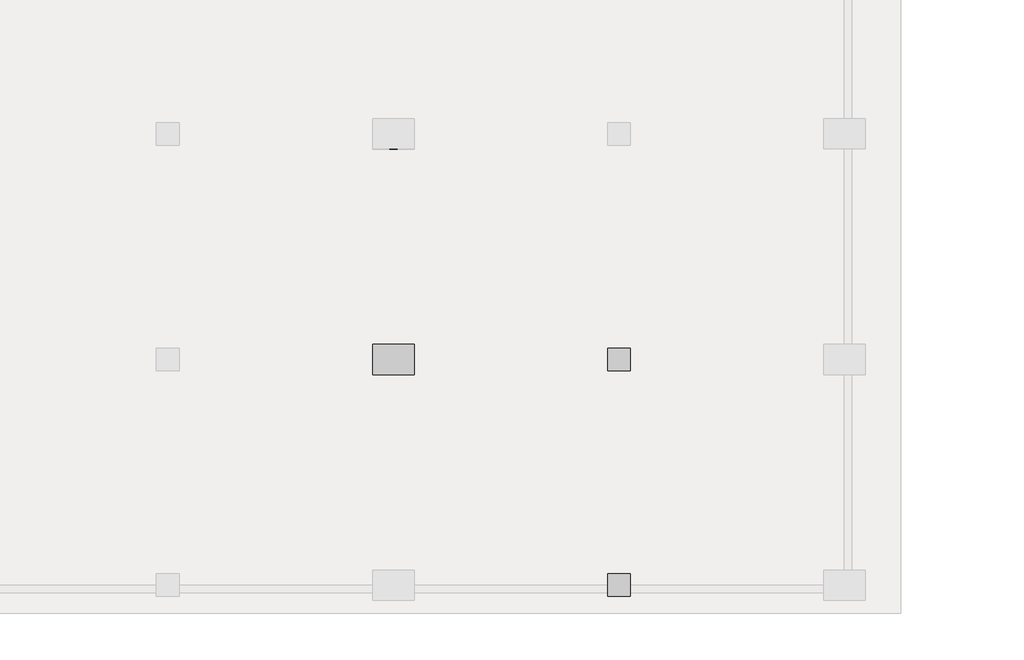
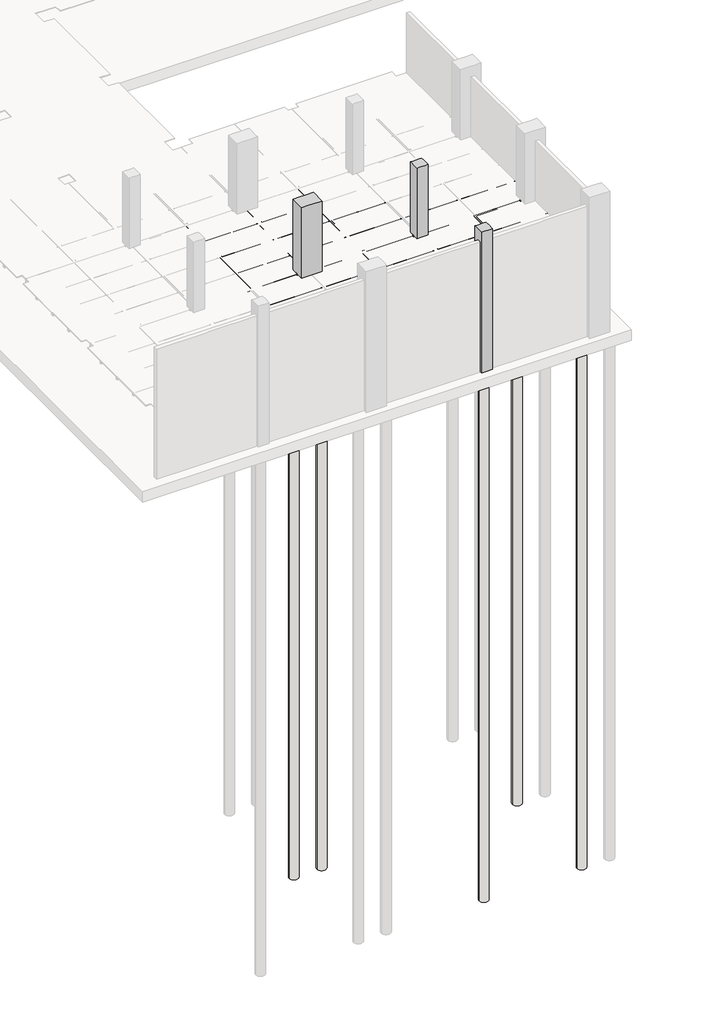
# Not in any storey, part 4 of 16: 30 beams, 5 slabs, 3 columns.
"""IFC4 building model written with IfcOpenShell, lengths in millimetres."""

from ifc_helpers import new_model, si_unit, point, frame, frame_2d, origin, place, context, project, spatial, polyline, circle_curve, trimmed, segment, composite_curve, outline, extrude, faceted_brep, element, save

model = new_model("IFC4")

# Units and contexts
model_context = context("Model", 3, world=origin())
ifc_project = project(units=[si_unit("LENGTHUNIT", "METRE", prefix="MILLI")], contexts=[model_context])

# Site, building
site = spatial("IfcSite", under=ifc_project)
building = spatial("IfcBuilding", under=site)

# Beams
placement = place(None, origin())
element("IfcBeam", 1, ObjectType="Steel Framing_H_KS : H_SB_AR_S02_H-400x200x8x13_BSG1", at=placement, inside=building, context=model_context, shape_type="SweptSolid", body=[
    extrude(outline(composite_curve([segment(polyline([(-53900.0, -4187.0381366), (-53900.0, -4200.0381366), (-54100.0, -4200.0381366), (-54100.0, -4187.0381366), (-54020.0, -4187.0381366)]), True, "CONTINUOUS"), segment(trimmed(circle_curve(frame_2d((-54020.0, -4171.0381366)), 16.0), [point((-54020.0, -4187.0381366))], [point((-54004.0, -4171.0381366))], True, "CARTESIAN"), True, "CONTINUOUS"), segment(polyline([(-54004.0, -4171.0381366), (-54004.0, -3829.0381366)]), True, "CONTINUOUS"), segment(trimmed(circle_curve(frame_2d((-54020.0, -3829.0381366)), 16.0), [point((-54004.0, -3829.0381366))], [point((-54020.0, -3813.0381366))], True, "CARTESIAN"), True, "CONTINUOUS"), segment(polyline([(-54020.0, -3813.0381366), (-54100.0, -3813.0381366), (-54100.0, -3800.0381366), (-53900.0, -3800.0381366), (-53900.0, -3813.0381366), (-53980.0, -3813.0381366)]), True, "CONTINUOUS"), segment(trimmed(circle_curve(frame_2d((-53980.0, -3829.0381366)), 16.0), [point((-53980.0, -3813.0381366))], [point((-53996.0, -3829.0381366))], True, "CARTESIAN"), True, "CONTINUOUS"), segment(polyline([(-53996.0, -3829.0381366), (-53996.0, -4171.0381366)]), True, "CONTINUOUS"), segment(trimmed(circle_curve(frame_2d((-53980.0, -4171.0381366)), 16.0), [point((-53996.0, -4171.0381366))], [point((-53980.0, -4187.0381366))], True, "CARTESIAN"), True, "CONTINUOUS"), segment(polyline([(-53980.0, -4187.0381366), (-53900.0, -4187.0381366)]), True, "CONTINUOUS")], self_intersect=False)), frame((30312.7, 0.0, 0.0), z_axis=(1.0, 0.0, 0.0), x_axis=(0.0, 1.0, 0.0)), (0.0, 0.0, 1.0), 5124.6),
])
element("IfcBeam", 2, ObjectType="Steel Framing_H_KS : H_SB_AR_S02_H-400x200x8x13_BSG2", at=placement, inside=building, context=model_context, shape_type="SweptSolid", body=[
    extrude(outline(composite_curve([segment(polyline([(-4187.0381366, 35900.0), (-4200.0381366, 35900.0), (-4200.0381366, 36100.0), (-4187.0381366, 36100.0), (-4187.0381366, 36020.0)]), True, "CONTINUOUS"), segment(trimmed(circle_curve(frame_2d((-4171.0381366, 36020.0)), 16.0), [point((-4187.0381366, 36020.0))], [point((-4171.0381366, 36004.0))], True, "CARTESIAN"), True, "CONTINUOUS"), segment(polyline([(-4171.0381366, 36004.0), (-3829.0381366, 36004.0)]), True, "CONTINUOUS"), segment(trimmed(circle_curve(frame_2d((-3829.0381366, 36020.0)), 16.0), [point((-3829.0381366, 36004.0))], [point((-3813.0381366, 36020.0))], True, "CARTESIAN"), True, "CONTINUOUS"), segment(polyline([(-3813.0381366, 36020.0), (-3813.0381366, 36100.0), (-3800.0381366, 36100.0), (-3800.0381366, 35900.0), (-3813.0381366, 35900.0), (-3813.0381366, 35980.0)]), True, "CONTINUOUS"), segment(trimmed(circle_curve(frame_2d((-3829.0381366, 35980.0)), 16.0), [point((-3813.0381366, 35980.0))], [point((-3829.0381366, 35996.0))], True, "CARTESIAN"), True, "CONTINUOUS"), segment(polyline([(-3829.0381366, 35996.0), (-4171.0381366, 35996.0)]), True, "CONTINUOUS"), segment(trimmed(circle_curve(frame_2d((-4171.0381366, 35980.0)), 16.0), [point((-4171.0381366, 35996.0))], [point((-4187.0381366, 35980.0))], True, "CARTESIAN"), True, "CONTINUOUS"), segment(polyline([(-4187.0381366, 35980.0), (-4187.0381366, 35900.0)]), True, "CONTINUOUS")], self_intersect=False)), frame((0.0, -53587.3, 0.0), z_axis=(0.0, 1.0, 0.0), x_axis=(0.0, 0.0, 1.0)), (0.0, 0.0, 1.0), 5174.6),
])
element("IfcBeam", 3, ObjectType="Steel Framing_H_KS : H_SB_AR_S02_H-400x200x8x13_BSB1", at=placement, inside=building, context=model_context, shape_type="SweptSolid", body=[
    extrude(outline(composite_curve([segment(polyline([(-4187.0381366, 32900.0), (-4200.0381366, 32900.0), (-4200.0381366, 33100.0), (-4187.0381366, 33100.0), (-4187.0381366, 33020.0)]), True, "CONTINUOUS"), segment(trimmed(circle_curve(frame_2d((-4171.0381366, 33020.0)), 16.0), [point((-4187.0381366, 33020.0))], [point((-4171.0381366, 33004.0))], True, "CARTESIAN"), True, "CONTINUOUS"), segment(polyline([(-4171.0381366, 33004.0), (-3829.0381366, 33004.0)]), True, "CONTINUOUS"), segment(trimmed(circle_curve(frame_2d((-3829.0381366, 33020.0)), 16.0), [point((-3829.0381366, 33004.0))], [point((-3813.0381366, 33020.0))], True, "CARTESIAN"), True, "CONTINUOUS"), segment(polyline([(-3813.0381366, 33020.0), (-3813.0381366, 33100.0), (-3800.0381366, 33100.0), (-3800.0381366, 32900.0), (-3813.0381366, 32900.0), (-3813.0381366, 32980.0)]), True, "CONTINUOUS"), segment(trimmed(circle_curve(frame_2d((-3829.0381366, 32980.0)), 16.0), [point((-3813.0381366, 32980.0))], [point((-3829.0381366, 32996.0))], True, "CARTESIAN"), True, "CONTINUOUS"), segment(polyline([(-3829.0381366, 32996.0), (-4171.0381366, 32996.0)]), True, "CONTINUOUS"), segment(trimmed(circle_curve(frame_2d((-4171.0381366, 32980.0)), 16.0), [point((-4171.0381366, 32996.0))], [point((-4187.0381366, 32980.0))], True, "CARTESIAN"), True, "CONTINUOUS"), segment(polyline([(-4187.0381366, 32980.0), (-4187.0381366, 32900.0)]), True, "CONTINUOUS")], self_intersect=False)), frame((0.0, -53887.3, 0.0), z_axis=(0.0, 1.0, 0.0), x_axis=(0.0, 0.0, 1.0)), (0.0, 0.0, 1.0), 5774.6),
])
element("IfcBeam", 4, ObjectType="Steel Framing_C_KS : H_SB_AR_S02_C-150x75x6.5x10_J1", at=placement, inside=building, context=model_context, shape_type="SweptSolid", body=[
    extrude(outline(composite_curve([segment(polyline([(-50977.2, -3800.0381366), (-50977.2, -3950.0381366), (-51052.2, -3950.0381366)]), True, "CONTINUOUS"), segment(trimmed(circle_curve(frame_2d((-51042.2, -3950.0381366)), 10.0), [point((-51052.2, -3950.0381366))], [point((-51042.2, -3940.0381366))], False, "CARTESIAN"), True, "CONTINUOUS"), segment(polyline([(-51042.2, -3940.0381366), (-50983.7, -3930.7726469), (-50983.7, -3819.3036264), (-51042.2, -3810.0381366)]), True, "CONTINUOUS"), segment(trimmed(circle_curve(frame_2d((-51042.2, -3800.0381366)), 10.0), [point((-51042.2, -3810.0381366))], [point((-51052.2, -3800.0381366))], False, "CARTESIAN"), True, "CONTINUOUS"), segment(polyline([(-51052.2, -3800.0381366), (-50977.2, -3800.0381366)]), True, "CONTINUOUS")], self_intersect=False)), frame((33112.7, 0.0, 0.0), z_axis=(1.0, 0.0, 0.0), x_axis=(0.0, 1.0, 0.0)), (0.0, 0.0, 1.0), 2774.6),
])
element("IfcBeam", 5, ObjectType="Steel Framing_C_KS : H_SB_AR_S02_C-150x75x6.5x10_J1", at=placement, inside=building, context=model_context, shape_type="SweptSolid", body=[
    extrude(outline(composite_curve([segment(polyline([(-52477.2, -3800.0381366), (-52477.2, -3950.0381366), (-52552.2, -3950.0381366)]), True, "CONTINUOUS"), segment(trimmed(circle_curve(frame_2d((-52542.2, -3950.0381366)), 10.0), [point((-52552.2, -3950.0381366))], [point((-52542.2, -3940.0381366))], False, "CARTESIAN"), True, "CONTINUOUS"), segment(polyline([(-52542.2, -3940.0381366), (-52483.7, -3930.7726469), (-52483.7, -3819.3036264), (-52542.2, -3810.0381366)]), True, "CONTINUOUS"), segment(trimmed(circle_curve(frame_2d((-52542.2, -3800.0381366)), 10.0), [point((-52542.2, -3810.0381366))], [point((-52552.2, -3800.0381366))], False, "CARTESIAN"), True, "CONTINUOUS"), segment(polyline([(-52552.2, -3800.0381366), (-52477.2, -3800.0381366)]), True, "CONTINUOUS")], self_intersect=False)), frame((33112.7, 0.0, 0.0), z_axis=(1.0, 0.0, 0.0), x_axis=(0.0, 1.0, 0.0)), (0.0, 0.0, 1.0), 2774.6),
])
element("IfcBeam", 6, ObjectType="Steel Framing_C_KS : H_SB_AR_S02_C-150x75x6.5x10_J1", at=placement, inside=building, context=model_context, shape_type="SweptSolid", body=[
    extrude(outline(composite_curve([segment(polyline([(-49477.2, -3800.0381366), (-49477.2, -3950.0381366), (-49552.2, -3950.0381366)]), True, "CONTINUOUS"), segment(trimmed(circle_curve(frame_2d((-49542.2, -3950.0381366)), 10.0), [point((-49552.2, -3950.0381366))], [point((-49542.2, -3940.0381366))], False, "CARTESIAN"), True, "CONTINUOUS"), segment(polyline([(-49542.2, -3940.0381366), (-49483.7, -3930.7726469), (-49483.7, -3819.3036264), (-49542.2, -3810.0381366)]), True, "CONTINUOUS"), segment(trimmed(circle_curve(frame_2d((-49542.2, -3800.0381366)), 10.0), [point((-49542.2, -3810.0381366))], [point((-49552.2, -3800.0381366))], False, "CARTESIAN"), True, "CONTINUOUS"), segment(polyline([(-49552.2, -3800.0381366), (-49477.2, -3800.0381366)]), True, "CONTINUOUS")], self_intersect=False)), frame((33112.7, 0.0, 0.0), z_axis=(1.0, 0.0, 0.0), x_axis=(0.0, 1.0, 0.0)), (0.0, 0.0, 1.0), 2774.6),
])
element("IfcBeam", 7, ObjectType="Steel Framing_H_KS : H_SB_AR_S02_H-400x200x8x13_BSG1", at=placement, inside=building, context=model_context, shape_type="SweptSolid", body=[
    extrude(outline(composite_curve([segment(polyline([(-53900.0, -4187.0381366), (-53900.0, -4200.0381366), (-54100.0, -4200.0381366), (-54100.0, -4187.0381366), (-54020.0, -4187.0381366)]), True, "CONTINUOUS"), segment(trimmed(circle_curve(frame_2d((-54020.0, -4171.0381366)), 16.0), [point((-54020.0, -4187.0381366))], [point((-54004.0, -4171.0381366))], True, "CARTESIAN"), True, "CONTINUOUS"), segment(polyline([(-54004.0, -4171.0381366), (-54004.0, -3829.0381366)]), True, "CONTINUOUS"), segment(trimmed(circle_curve(frame_2d((-54020.0, -3829.0381366)), 16.0), [point((-54004.0, -3829.0381366))], [point((-54020.0, -3813.0381366))], True, "CARTESIAN"), True, "CONTINUOUS"), segment(polyline([(-54020.0, -3813.0381366), (-54100.0, -3813.0381366), (-54100.0, -3800.0381366), (-53900.0, -3800.0381366), (-53900.0, -3813.0381366), (-53980.0, -3813.0381366)]), True, "CONTINUOUS"), segment(trimmed(circle_curve(frame_2d((-53980.0, -3829.0381366)), 16.0), [point((-53980.0, -3813.0381366))], [point((-53996.0, -3829.0381366))], True, "CARTESIAN"), True, "CONTINUOUS"), segment(polyline([(-53996.0, -3829.0381366), (-53996.0, -4171.0381366)]), True, "CONTINUOUS"), segment(trimmed(circle_curve(frame_2d((-53980.0, -4171.0381366)), 16.0), [point((-53996.0, -4171.0381366))], [point((-53980.0, -4187.0381366))], True, "CARTESIAN"), True, "CONTINUOUS"), segment(polyline([(-53980.0, -4187.0381366), (-53900.0, -4187.0381366)]), True, "CONTINUOUS")], self_intersect=False)), frame((36562.7, 0.0, 0.0), z_axis=(1.0, 0.0, 0.0), x_axis=(0.0, 1.0, 0.0)), (0.0, 0.0, 1.0), 5124.6),
])
element("IfcBeam", 8, ObjectType="Steel Framing_H_KS : H_SB_AR_S02_H-400x200x8x13_BSB1", at=placement, inside=building, context=model_context, shape_type="SweptSolid", body=[
    extrude(outline(composite_curve([segment(polyline([(-4187.0381366, 38900.0), (-4200.0381366, 38900.0), (-4200.0381366, 39100.0), (-4187.0381366, 39100.0), (-4187.0381366, 39020.0)]), True, "CONTINUOUS"), segment(trimmed(circle_curve(frame_2d((-4171.0381366, 39020.0)), 16.0), [point((-4187.0381366, 39020.0))], [point((-4171.0381366, 39004.0))], True, "CARTESIAN"), True, "CONTINUOUS"), segment(polyline([(-4171.0381366, 39004.0), (-3829.0381366, 39004.0)]), True, "CONTINUOUS"), segment(trimmed(circle_curve(frame_2d((-3829.0381366, 39020.0)), 16.0), [point((-3829.0381366, 39004.0))], [point((-3813.0381366, 39020.0))], True, "CARTESIAN"), True, "CONTINUOUS"), segment(polyline([(-3813.0381366, 39020.0), (-3813.0381366, 39100.0), (-3800.0381366, 39100.0), (-3800.0381366, 38900.0), (-3813.0381366, 38900.0), (-3813.0381366, 38980.0)]), True, "CONTINUOUS"), segment(trimmed(circle_curve(frame_2d((-3829.0381366, 38980.0)), 16.0), [point((-3813.0381366, 38980.0))], [point((-3829.0381366, 38996.0))], True, "CARTESIAN"), True, "CONTINUOUS"), segment(polyline([(-3829.0381366, 38996.0), (-4171.0381366, 38996.0)]), True, "CONTINUOUS"), segment(trimmed(circle_curve(frame_2d((-4171.0381366, 38980.0)), 16.0), [point((-4171.0381366, 38996.0))], [point((-4187.0381366, 38980.0))], True, "CARTESIAN"), True, "CONTINUOUS"), segment(polyline([(-4187.0381366, 38980.0), (-4187.0381366, 38900.0)]), True, "CONTINUOUS")], self_intersect=False)), frame((0.0, -53887.3, 0.0), z_axis=(0.0, 1.0, 0.0), x_axis=(0.0, 0.0, 1.0)), (0.0, 0.0, 1.0), 5774.6),
])
element("IfcBeam", 9, ObjectType="Steel Framing_C_KS : H_SB_AR_S02_C-150x75x6.5x10_J1", at=placement, inside=building, context=model_context, shape_type="SweptSolid", body=[
    extrude(outline(composite_curve([segment(polyline([(-50977.2, -3800.0381366), (-50977.2, -3950.0381366), (-51052.2, -3950.0381366)]), True, "CONTINUOUS"), segment(trimmed(circle_curve(frame_2d((-51042.2, -3950.0381366)), 10.0), [point((-51052.2, -3950.0381366))], [point((-51042.2, -3940.0381366))], False, "CARTESIAN"), True, "CONTINUOUS"), segment(polyline([(-51042.2, -3940.0381366), (-50983.7, -3930.7726469), (-50983.7, -3819.3036264), (-51042.2, -3810.0381366)]), True, "CONTINUOUS"), segment(trimmed(circle_curve(frame_2d((-51042.2, -3800.0381366)), 10.0), [point((-51042.2, -3810.0381366))], [point((-51052.2, -3800.0381366))], False, "CARTESIAN"), True, "CONTINUOUS"), segment(polyline([(-51052.2, -3800.0381366), (-50977.2, -3800.0381366)]), True, "CONTINUOUS")], self_intersect=False)), frame((36112.7, 0.0, 0.0), z_axis=(1.0, 0.0, 0.0), x_axis=(0.0, 1.0, 0.0)), (0.0, 0.0, 1.0), 2774.6),
])
element("IfcBeam", 10, ObjectType="Steel Framing_C_KS : H_SB_AR_S02_C-150x75x6.5x10_J1", at=placement, inside=building, context=model_context, shape_type="SweptSolid", body=[
    extrude(outline(composite_curve([segment(polyline([(-52477.2, -3800.0381366), (-52477.2, -3950.0381366), (-52552.2, -3950.0381366)]), True, "CONTINUOUS"), segment(trimmed(circle_curve(frame_2d((-52542.2, -3950.0381366)), 10.0), [point((-52552.2, -3950.0381366))], [point((-52542.2, -3940.0381366))], False, "CARTESIAN"), True, "CONTINUOUS"), segment(polyline([(-52542.2, -3940.0381366), (-52483.7, -3930.7726469), (-52483.7, -3819.3036264), (-52542.2, -3810.0381366)]), True, "CONTINUOUS"), segment(trimmed(circle_curve(frame_2d((-52542.2, -3800.0381366)), 10.0), [point((-52542.2, -3810.0381366))], [point((-52552.2, -3800.0381366))], False, "CARTESIAN"), True, "CONTINUOUS"), segment(polyline([(-52552.2, -3800.0381366), (-52477.2, -3800.0381366)]), True, "CONTINUOUS")], self_intersect=False)), frame((36112.7, 0.0, 0.0), z_axis=(1.0, 0.0, 0.0), x_axis=(0.0, 1.0, 0.0)), (0.0, 0.0, 1.0), 2774.6),
])
element("IfcBeam", 11, ObjectType="Steel Framing_C_KS : H_SB_AR_S02_C-150x75x6.5x10_J1", at=placement, inside=building, context=model_context, shape_type="SweptSolid", body=[
    extrude(outline(composite_curve([segment(polyline([(-49477.2, -3800.0381366), (-49477.2, -3950.0381366), (-49552.2, -3950.0381366)]), True, "CONTINUOUS"), segment(trimmed(circle_curve(frame_2d((-49542.2, -3950.0381366)), 10.0), [point((-49552.2, -3950.0381366))], [point((-49542.2, -3940.0381366))], False, "CARTESIAN"), True, "CONTINUOUS"), segment(polyline([(-49542.2, -3940.0381366), (-49483.7, -3930.7726469), (-49483.7, -3819.3036264), (-49542.2, -3810.0381366)]), True, "CONTINUOUS"), segment(trimmed(circle_curve(frame_2d((-49542.2, -3800.0381366)), 10.0), [point((-49542.2, -3810.0381366))], [point((-49552.2, -3800.0381366))], False, "CARTESIAN"), True, "CONTINUOUS"), segment(polyline([(-49552.2, -3800.0381366), (-49477.2, -3800.0381366)]), True, "CONTINUOUS")], self_intersect=False)), frame((36112.7, 0.0, 0.0), z_axis=(1.0, 0.0, 0.0), x_axis=(0.0, 1.0, 0.0)), (0.0, 0.0, 1.0), 2774.6),
])
element("IfcBeam", 12, ObjectType="Steel Framing_C_KS : H_SB_AR_S02_C-150x75x6.5x10_J1", at=placement, inside=building, context=model_context, shape_type="SweptSolid", body=[
    extrude(outline(composite_curve([segment(polyline([(-50977.2, -3800.0381366), (-50977.2, -3950.0381366), (-51052.2, -3950.0381366)]), True, "CONTINUOUS"), segment(trimmed(circle_curve(frame_2d((-51042.2, -3950.0381366)), 10.0), [point((-51052.2, -3950.0381366))], [point((-51042.2, -3940.0381366))], False, "CARTESIAN"), True, "CONTINUOUS"), segment(polyline([(-51042.2, -3940.0381366), (-50983.7, -3930.7726469), (-50983.7, -3819.3036264), (-51042.2, -3810.0381366)]), True, "CONTINUOUS"), segment(trimmed(circle_curve(frame_2d((-51042.2, -3800.0381366)), 10.0), [point((-51042.2, -3810.0381366))], [point((-51052.2, -3800.0381366))], False, "CARTESIAN"), True, "CONTINUOUS"), segment(polyline([(-51052.2, -3800.0381366), (-50977.2, -3800.0381366)]), True, "CONTINUOUS")], self_intersect=False)), frame((39112.7, 0.0, 0.0), z_axis=(1.0, 0.0, 0.0), x_axis=(0.0, 1.0, 0.0)), (0.0, 0.0, 1.0), 2774.6),
])
element("IfcBeam", 13, ObjectType="Steel Framing_C_KS : H_SB_AR_S02_C-150x75x6.5x10_J1", at=placement, inside=building, context=model_context, shape_type="SweptSolid", body=[
    extrude(outline(composite_curve([segment(polyline([(-52477.2, -3800.0381366), (-52477.2, -3950.0381366), (-52552.2, -3950.0381366)]), True, "CONTINUOUS"), segment(trimmed(circle_curve(frame_2d((-52542.2, -3950.0381366)), 10.0), [point((-52552.2, -3950.0381366))], [point((-52542.2, -3940.0381366))], False, "CARTESIAN"), True, "CONTINUOUS"), segment(polyline([(-52542.2, -3940.0381366), (-52483.7, -3930.7726469), (-52483.7, -3819.3036264), (-52542.2, -3810.0381366)]), True, "CONTINUOUS"), segment(trimmed(circle_curve(frame_2d((-52542.2, -3800.0381366)), 10.0), [point((-52542.2, -3810.0381366))], [point((-52552.2, -3800.0381366))], False, "CARTESIAN"), True, "CONTINUOUS"), segment(polyline([(-52552.2, -3800.0381366), (-52477.2, -3800.0381366)]), True, "CONTINUOUS")], self_intersect=False)), frame((39112.7, 0.0, 0.0), z_axis=(1.0, 0.0, 0.0), x_axis=(0.0, 1.0, 0.0)), (0.0, 0.0, 1.0), 2774.6),
])
element("IfcBeam", 14, ObjectType="Steel Framing_H_KS : H_SB_AR_S02_H-400x200x8x13_BSG1", at=placement, inside=building, context=model_context, shape_type="SweptSolid", body=[
    extrude(outline(composite_curve([segment(polyline([(-53900.0, -4187.0381366), (-53900.0, -4200.0381366), (-54100.0, -4200.0381366), (-54100.0, -4187.0381366), (-54020.0, -4187.0381366)]), True, "CONTINUOUS"), segment(trimmed(circle_curve(frame_2d((-54020.0, -4171.0381366)), 16.0), [point((-54020.0, -4187.0381366))], [point((-54004.0, -4171.0381366))], True, "CARTESIAN"), True, "CONTINUOUS"), segment(polyline([(-54004.0, -4171.0381366), (-54004.0, -3829.0381366)]), True, "CONTINUOUS"), segment(trimmed(circle_curve(frame_2d((-54020.0, -3829.0381366)), 16.0), [point((-54004.0, -3829.0381366))], [point((-54020.0, -3813.0381366))], True, "CARTESIAN"), True, "CONTINUOUS"), segment(polyline([(-54020.0, -3813.0381366), (-54100.0, -3813.0381366), (-54100.0, -3800.0381366), (-53900.0, -3800.0381366), (-53900.0, -3813.0381366), (-53980.0, -3813.0381366)]), True, "CONTINUOUS"), segment(trimmed(circle_curve(frame_2d((-53980.0, -3829.0381366)), 16.0), [point((-53980.0, -3813.0381366))], [point((-53996.0, -3829.0381366))], True, "CARTESIAN"), True, "CONTINUOUS"), segment(polyline([(-53996.0, -3829.0381366), (-53996.0, -4171.0381366)]), True, "CONTINUOUS"), segment(trimmed(circle_curve(frame_2d((-53980.0, -4171.0381366)), 16.0), [point((-53996.0, -4171.0381366))], [point((-53980.0, -4187.0381366))], True, "CARTESIAN"), True, "CONTINUOUS"), segment(polyline([(-53980.0, -4187.0381366), (-53900.0, -4187.0381366)]), True, "CONTINUOUS")], self_intersect=False)), frame((42312.7, 0.0, 0.0), z_axis=(1.0, 0.0, 0.0), x_axis=(0.0, 1.0, 0.0)), (0.0, 0.0, 1.0), 5124.6),
])
element("IfcBeam", 15, ObjectType="Steel Framing_C_KS : H_SB_AR_S02_C-150x75x6.5x10_J1", at=placement, inside=building, context=model_context, shape_type="SweptSolid", body=[
    extrude(outline(composite_curve([segment(polyline([(-52477.2, -3800.0381366), (-52477.2, -3950.0381366), (-52552.2, -3950.0381366)]), True, "CONTINUOUS"), segment(trimmed(circle_curve(frame_2d((-52542.2, -3950.0381366)), 10.0), [point((-52552.2, -3950.0381366))], [point((-52542.2, -3940.0381366))], False, "CARTESIAN"), True, "CONTINUOUS"), segment(polyline([(-52542.2, -3940.0381366), (-52483.7, -3930.7726469), (-52483.7, -3819.3036264), (-52542.2, -3810.0381366)]), True, "CONTINUOUS"), segment(trimmed(circle_curve(frame_2d((-52542.2, -3800.0381366)), 10.0), [point((-52542.2, -3810.0381366))], [point((-52552.2, -3800.0381366))], False, "CARTESIAN"), True, "CONTINUOUS"), segment(polyline([(-52552.2, -3800.0381366), (-52477.2, -3800.0381366)]), True, "CONTINUOUS")], self_intersect=False)), frame((42112.7, 0.0, 0.0), z_axis=(1.0, 0.0, 0.0), x_axis=(0.0, 1.0, 0.0)), (0.0, 0.0, 1.0), 2774.6),
])
element("IfcBeam", 16, ObjectType="Steel Framing_C_KS : H_SB_AR_S02_C-150x75x6.5x10_J1", at=placement, inside=building, context=model_context, shape_type="SweptSolid", body=[
    extrude(outline(composite_curve([segment(polyline([(-52477.2, -3800.0381366), (-52477.2, -3950.0381366), (-52552.2, -3950.0381366)]), True, "CONTINUOUS"), segment(trimmed(circle_curve(frame_2d((-52542.2, -3950.0381366)), 10.0), [point((-52552.2, -3950.0381366))], [point((-52542.2, -3940.0381366))], False, "CARTESIAN"), True, "CONTINUOUS"), segment(polyline([(-52542.2, -3940.0381366), (-52483.7, -3930.7726469), (-52483.7, -3819.3036264), (-52542.2, -3810.0381366)]), True, "CONTINUOUS"), segment(trimmed(circle_curve(frame_2d((-52542.2, -3800.0381366)), 10.0), [point((-52542.2, -3810.0381366))], [point((-52552.2, -3800.0381366))], False, "CARTESIAN"), True, "CONTINUOUS"), segment(polyline([(-52552.2, -3800.0381366), (-52477.2, -3800.0381366)]), True, "CONTINUOUS")], self_intersect=False)), frame((45112.7, 0.0, 0.0), z_axis=(1.0, 0.0, 0.0), x_axis=(0.0, 1.0, 0.0)), (0.0, 0.0, 1.0), 2887.3),
])
element("IfcBeam", 17, ObjectType="Steel Framing_C_KS : H_SB_AR_S02_C-150x75x6.5x10_J1", at=placement, inside=building, context=model_context, shape_type="SweptSolid", body=[
    extrude(outline(composite_curve([segment(polyline([(-55477.2, -3800.0381366), (-55477.2, -3950.0381366), (-55552.2, -3950.0381366)]), True, "CONTINUOUS"), segment(trimmed(circle_curve(frame_2d((-55542.2, -3950.0381366)), 10.0), [point((-55552.2, -3950.0381366))], [point((-55542.2, -3940.0381366))], False, "CARTESIAN"), True, "CONTINUOUS"), segment(polyline([(-55542.2, -3940.0381366), (-55483.7, -3930.7726469), (-55483.7, -3819.3036264), (-55542.2, -3810.0381366)]), True, "CONTINUOUS"), segment(trimmed(circle_curve(frame_2d((-55542.2, -3800.0381366)), 10.0), [point((-55542.2, -3810.0381366))], [point((-55552.2, -3800.0381366))], False, "CARTESIAN"), True, "CONTINUOUS"), segment(polyline([(-55552.2, -3800.0381366), (-55477.2, -3800.0381366)]), True, "CONTINUOUS")], self_intersect=False)), frame((33112.7, 0.0, 0.0), z_axis=(1.0, 0.0, 0.0), x_axis=(0.0, 1.0, 0.0)), (0.0, 0.0, 1.0), 2774.6),
])
element("IfcBeam", 18, ObjectType="Steel Framing_H_KS : H_SB_AR_S02_H-400x200x8x13_BSG2", at=placement, inside=building, context=model_context, shape_type="SweptSolid", body=[
    extrude(outline(composite_curve([segment(polyline([(-4187.0381366, 41900.0), (-4200.0381366, 41900.0), (-4200.0381366, 42100.0), (-4187.0381366, 42100.0), (-4187.0381366, 42020.0)]), True, "CONTINUOUS"), segment(trimmed(circle_curve(frame_2d((-4171.0381366, 42020.0)), 16.0), [point((-4187.0381366, 42020.0))], [point((-4171.0381366, 42004.0))], True, "CARTESIAN"), True, "CONTINUOUS"), segment(polyline([(-4171.0381366, 42004.0), (-3829.0381366, 42004.0)]), True, "CONTINUOUS"), segment(trimmed(circle_curve(frame_2d((-3829.0381366, 42020.0)), 16.0), [point((-3829.0381366, 42004.0))], [point((-3813.0381366, 42020.0))], True, "CARTESIAN"), True, "CONTINUOUS"), segment(polyline([(-3813.0381366, 42020.0), (-3813.0381366, 42100.0), (-3800.0381366, 42100.0), (-3800.0381366, 41900.0), (-3813.0381366, 41900.0), (-3813.0381366, 41980.0)]), True, "CONTINUOUS"), segment(trimmed(circle_curve(frame_2d((-3829.0381366, 41980.0)), 16.0), [point((-3813.0381366, 41980.0))], [point((-3829.0381366, 41996.0))], True, "CARTESIAN"), True, "CONTINUOUS"), segment(polyline([(-3829.0381366, 41996.0), (-4171.0381366, 41996.0)]), True, "CONTINUOUS"), segment(trimmed(circle_curve(frame_2d((-4171.0381366, 41980.0)), 16.0), [point((-4171.0381366, 41996.0))], [point((-4187.0381366, 41980.0))], True, "CARTESIAN"), True, "CONTINUOUS"), segment(polyline([(-4187.0381366, 41980.0), (-4187.0381366, 41900.0)]), True, "CONTINUOUS")], self_intersect=False)), frame((0.0, -59687.3, 0.0), z_axis=(0.0, 1.0, 0.0), x_axis=(0.0, 0.0, 1.0)), (0.0, 0.0, 1.0), 5374.6),
])
element("IfcBeam", 19, ObjectType="Steel Framing_H_KS : H_SB_AR_S02_H-400x200x8x13_BSB1", at=placement, inside=building, context=model_context, shape_type="SweptSolid", body=[
    extrude(outline(composite_curve([segment(polyline([(-4187.0381366, 38900.0), (-4200.0381366, 38900.0), (-4200.0381366, 39100.0), (-4187.0381366, 39100.0), (-4187.0381366, 39020.0)]), True, "CONTINUOUS"), segment(trimmed(circle_curve(frame_2d((-4171.0381366, 39020.0)), 16.0), [point((-4187.0381366, 39020.0))], [point((-4171.0381366, 39004.0))], True, "CARTESIAN"), True, "CONTINUOUS"), segment(polyline([(-4171.0381366, 39004.0), (-3829.0381366, 39004.0)]), True, "CONTINUOUS"), segment(trimmed(circle_curve(frame_2d((-3829.0381366, 39020.0)), 16.0), [point((-3829.0381366, 39004.0))], [point((-3813.0381366, 39020.0))], True, "CARTESIAN"), True, "CONTINUOUS"), segment(polyline([(-3813.0381366, 39020.0), (-3813.0381366, 39100.0), (-3800.0381366, 39100.0), (-3800.0381366, 38900.0), (-3813.0381366, 38900.0), (-3813.0381366, 38980.0)]), True, "CONTINUOUS"), segment(trimmed(circle_curve(frame_2d((-3829.0381366, 38980.0)), 16.0), [point((-3813.0381366, 38980.0))], [point((-3829.0381366, 38996.0))], True, "CARTESIAN"), True, "CONTINUOUS"), segment(polyline([(-3829.0381366, 38996.0), (-4171.0381366, 38996.0)]), True, "CONTINUOUS"), segment(trimmed(circle_curve(frame_2d((-4171.0381366, 38980.0)), 16.0), [point((-4171.0381366, 38996.0))], [point((-4187.0381366, 38980.0))], True, "CARTESIAN"), True, "CONTINUOUS"), segment(polyline([(-4187.0381366, 38980.0), (-4187.0381366, 38900.0)]), True, "CONTINUOUS")], self_intersect=False)), frame((0.0, -60000.0, 0.0), z_axis=(0.0, 1.0, 0.0), x_axis=(0.0, 0.0, 1.0)), (0.0, 0.0, 1.0), 5887.3),
])
element("IfcBeam", 20, ObjectType="Steel Framing_C_KS : H_SB_AR_S02_C-150x75x6.5x10_J1", at=placement, inside=building, context=model_context, shape_type="SweptSolid", body=[
    extrude(outline(composite_curve([segment(polyline([(-55477.2, -3800.0381366), (-55477.2, -3950.0381366), (-55552.2, -3950.0381366)]), True, "CONTINUOUS"), segment(trimmed(circle_curve(frame_2d((-55542.2, -3950.0381366)), 10.0), [point((-55552.2, -3950.0381366))], [point((-55542.2, -3940.0381366))], False, "CARTESIAN"), True, "CONTINUOUS"), segment(polyline([(-55542.2, -3940.0381366), (-55483.7, -3930.7726469), (-55483.7, -3819.3036264), (-55542.2, -3810.0381366)]), True, "CONTINUOUS"), segment(trimmed(circle_curve(frame_2d((-55542.2, -3800.0381366)), 10.0), [point((-55542.2, -3810.0381366))], [point((-55552.2, -3800.0381366))], False, "CARTESIAN"), True, "CONTINUOUS"), segment(polyline([(-55552.2, -3800.0381366), (-55477.2, -3800.0381366)]), True, "CONTINUOUS")], self_intersect=False)), frame((36112.7, 0.0, 0.0), z_axis=(1.0, 0.0, 0.0), x_axis=(0.0, 1.0, 0.0)), (0.0, 0.0, 1.0), 2774.6),
])
element("IfcBeam", 21, ObjectType="Steel Framing_C_KS : H_SB_AR_S02_C-150x75x6.5x10_J1", at=placement, inside=building, context=model_context, shape_type="SweptSolid", body=[
    extrude(outline(composite_curve([segment(polyline([(-56977.2, -3800.0381366), (-56977.2, -3950.0381366), (-57052.2, -3950.0381366)]), True, "CONTINUOUS"), segment(trimmed(circle_curve(frame_2d((-57042.2, -3950.0381366)), 10.0), [point((-57052.2, -3950.0381366))], [point((-57042.2, -3940.0381366))], False, "CARTESIAN"), True, "CONTINUOUS"), segment(polyline([(-57042.2, -3940.0381366), (-56983.7, -3930.7726469), (-56983.7, -3819.3036264), (-57042.2, -3810.0381366)]), True, "CONTINUOUS"), segment(trimmed(circle_curve(frame_2d((-57042.2, -3800.0381366)), 10.0), [point((-57042.2, -3810.0381366))], [point((-57052.2, -3800.0381366))], False, "CARTESIAN"), True, "CONTINUOUS"), segment(polyline([(-57052.2, -3800.0381366), (-56977.2, -3800.0381366)]), True, "CONTINUOUS")], self_intersect=False)), frame((39112.7, 0.0, 0.0), z_axis=(1.0, 0.0, 0.0), x_axis=(0.0, 1.0, 0.0)), (0.0, 0.0, 1.0), 2774.6),
])
element("IfcBeam", 22, ObjectType="Steel Framing_C_KS : H_SB_AR_S02_C-150x75x6.5x10_J1", at=placement, inside=building, context=model_context, shape_type="SweptSolid", body=[
    extrude(outline(composite_curve([segment(polyline([(-58477.2, -3800.0381366), (-58477.2, -3950.0381366), (-58552.2, -3950.0381366)]), True, "CONTINUOUS"), segment(trimmed(circle_curve(frame_2d((-58542.2, -3950.0381366)), 10.0), [point((-58552.2, -3950.0381366))], [point((-58542.2, -3940.0381366))], False, "CARTESIAN"), True, "CONTINUOUS"), segment(polyline([(-58542.2, -3940.0381366), (-58483.7, -3930.7726469), (-58483.7, -3819.3036264), (-58542.2, -3810.0381366)]), True, "CONTINUOUS"), segment(trimmed(circle_curve(frame_2d((-58542.2, -3800.0381366)), 10.0), [point((-58542.2, -3810.0381366))], [point((-58552.2, -3800.0381366))], False, "CARTESIAN"), True, "CONTINUOUS"), segment(polyline([(-58552.2, -3800.0381366), (-58477.2, -3800.0381366)]), True, "CONTINUOUS")], self_intersect=False)), frame((39112.7, 0.0, 0.0), z_axis=(1.0, 0.0, 0.0), x_axis=(0.0, 1.0, 0.0)), (0.0, 0.0, 1.0), 2774.6),
])
element("IfcBeam", 23, ObjectType="Steel Framing_C_KS : H_SB_AR_S02_C-150x75x6.5x10_J1", at=placement, inside=building, context=model_context, shape_type="SweptSolid", body=[
    extrude(outline(composite_curve([segment(polyline([(-55477.2, -3800.0381366), (-55477.2, -3950.0381366), (-55552.2, -3950.0381366)]), True, "CONTINUOUS"), segment(trimmed(circle_curve(frame_2d((-55542.2, -3950.0381366)), 10.0), [point((-55552.2, -3950.0381366))], [point((-55542.2, -3940.0381366))], False, "CARTESIAN"), True, "CONTINUOUS"), segment(polyline([(-55542.2, -3940.0381366), (-55483.7, -3930.7726469), (-55483.7, -3819.3036264), (-55542.2, -3810.0381366)]), True, "CONTINUOUS"), segment(trimmed(circle_curve(frame_2d((-55542.2, -3800.0381366)), 10.0), [point((-55542.2, -3810.0381366))], [point((-55552.2, -3800.0381366))], False, "CARTESIAN"), True, "CONTINUOUS"), segment(polyline([(-55552.2, -3800.0381366), (-55477.2, -3800.0381366)]), True, "CONTINUOUS")], self_intersect=False)), frame((39112.7, 0.0, 0.0), z_axis=(1.0, 0.0, 0.0), x_axis=(0.0, 1.0, 0.0)), (0.0, 0.0, 1.0), 2774.6),
])
element("IfcBeam", 24, ObjectType="Steel Framing_H_KS : H_SB_AR_S02_H-400x200x8x13_BSB1", at=placement, inside=building, context=model_context, shape_type="SweptSolid", body=[
    extrude(outline(composite_curve([segment(polyline([(-4187.0381366, 44900.0), (-4200.0381366, 44900.0), (-4200.0381366, 45100.0), (-4187.0381366, 45100.0), (-4187.0381366, 45020.0)]), True, "CONTINUOUS"), segment(trimmed(circle_curve(frame_2d((-4171.0381366, 45020.0)), 16.0), [point((-4187.0381366, 45020.0))], [point((-4171.0381366, 45004.0))], True, "CARTESIAN"), True, "CONTINUOUS"), segment(polyline([(-4171.0381366, 45004.0), (-3829.0381366, 45004.0)]), True, "CONTINUOUS"), segment(trimmed(circle_curve(frame_2d((-3829.0381366, 45020.0)), 16.0), [point((-3829.0381366, 45004.0))], [point((-3813.0381366, 45020.0))], True, "CARTESIAN"), True, "CONTINUOUS"), segment(polyline([(-3813.0381366, 45020.0), (-3813.0381366, 45100.0), (-3800.0381366, 45100.0), (-3800.0381366, 44900.0), (-3813.0381366, 44900.0), (-3813.0381366, 44980.0)]), True, "CONTINUOUS"), segment(trimmed(circle_curve(frame_2d((-3829.0381366, 44980.0)), 16.0), [point((-3813.0381366, 44980.0))], [point((-3829.0381366, 44996.0))], True, "CARTESIAN"), True, "CONTINUOUS"), segment(polyline([(-3829.0381366, 44996.0), (-4171.0381366, 44996.0)]), True, "CONTINUOUS"), segment(trimmed(circle_curve(frame_2d((-4171.0381366, 44980.0)), 16.0), [point((-4171.0381366, 44996.0))], [point((-4187.0381366, 44980.0))], True, "CARTESIAN"), True, "CONTINUOUS"), segment(polyline([(-4187.0381366, 44980.0), (-4187.0381366, 44900.0)]), True, "CONTINUOUS")], self_intersect=False)), frame((0.0, -60000.0, 0.0), z_axis=(0.0, 1.0, 0.0), x_axis=(0.0, 0.0, 1.0)), (0.0, 0.0, 1.0), 5887.3),
])
element("IfcBeam", 25, ObjectType="Steel Framing_C_KS : H_SB_AR_S02_C-150x75x6.5x10_J1", at=placement, inside=building, context=model_context, shape_type="SweptSolid", body=[
    extrude(outline(composite_curve([segment(polyline([(-56977.2, -3800.0381366), (-56977.2, -3950.0381366), (-57052.2, -3950.0381366)]), True, "CONTINUOUS"), segment(trimmed(circle_curve(frame_2d((-57042.2, -3950.0381366)), 10.0), [point((-57052.2, -3950.0381366))], [point((-57042.2, -3940.0381366))], False, "CARTESIAN"), True, "CONTINUOUS"), segment(polyline([(-57042.2, -3940.0381366), (-56983.7, -3930.7726469), (-56983.7, -3819.3036264), (-57042.2, -3810.0381366)]), True, "CONTINUOUS"), segment(trimmed(circle_curve(frame_2d((-57042.2, -3800.0381366)), 10.0), [point((-57042.2, -3810.0381366))], [point((-57052.2, -3800.0381366))], False, "CARTESIAN"), True, "CONTINUOUS"), segment(polyline([(-57052.2, -3800.0381366), (-56977.2, -3800.0381366)]), True, "CONTINUOUS")], self_intersect=False)), frame((42112.7, 0.0, 0.0), z_axis=(1.0, 0.0, 0.0), x_axis=(0.0, 1.0, 0.0)), (0.0, 0.0, 1.0), 2774.6),
])
element("IfcBeam", 26, ObjectType="Steel Framing_C_KS : H_SB_AR_S02_C-150x75x6.5x10_J1", at=placement, inside=building, context=model_context, shape_type="SweptSolid", body=[
    extrude(outline(composite_curve([segment(polyline([(-58477.2, -3800.0381366), (-58477.2, -3950.0381366), (-58552.2, -3950.0381366)]), True, "CONTINUOUS"), segment(trimmed(circle_curve(frame_2d((-58542.2, -3950.0381366)), 10.0), [point((-58552.2, -3950.0381366))], [point((-58542.2, -3940.0381366))], False, "CARTESIAN"), True, "CONTINUOUS"), segment(polyline([(-58542.2, -3940.0381366), (-58483.7, -3930.7726469), (-58483.7, -3819.3036264), (-58542.2, -3810.0381366)]), True, "CONTINUOUS"), segment(trimmed(circle_curve(frame_2d((-58542.2, -3800.0381366)), 10.0), [point((-58542.2, -3810.0381366))], [point((-58552.2, -3800.0381366))], False, "CARTESIAN"), True, "CONTINUOUS"), segment(polyline([(-58552.2, -3800.0381366), (-58477.2, -3800.0381366)]), True, "CONTINUOUS")], self_intersect=False)), frame((42112.7, 0.0, 0.0), z_axis=(1.0, 0.0, 0.0), x_axis=(0.0, 1.0, 0.0)), (0.0, 0.0, 1.0), 2774.6),
])
element("IfcBeam", 27, ObjectType="Steel Framing_C_KS : H_SB_AR_S02_C-150x75x6.5x10_J1", at=placement, inside=building, context=model_context, shape_type="SweptSolid", body=[
    extrude(outline(composite_curve([segment(polyline([(-55477.2, -3800.0381366), (-55477.2, -3950.0381366), (-55552.2, -3950.0381366)]), True, "CONTINUOUS"), segment(trimmed(circle_curve(frame_2d((-55542.2, -3950.0381366)), 10.0), [point((-55552.2, -3950.0381366))], [point((-55542.2, -3940.0381366))], False, "CARTESIAN"), True, "CONTINUOUS"), segment(polyline([(-55542.2, -3940.0381366), (-55483.7, -3930.7726469), (-55483.7, -3819.3036264), (-55542.2, -3810.0381366)]), True, "CONTINUOUS"), segment(trimmed(circle_curve(frame_2d((-55542.2, -3800.0381366)), 10.0), [point((-55542.2, -3810.0381366))], [point((-55552.2, -3800.0381366))], False, "CARTESIAN"), True, "CONTINUOUS"), segment(polyline([(-55552.2, -3800.0381366), (-55477.2, -3800.0381366)]), True, "CONTINUOUS")], self_intersect=False)), frame((42112.7, 0.0, 0.0), z_axis=(1.0, 0.0, 0.0), x_axis=(0.0, 1.0, 0.0)), (0.0, 0.0, 1.0), 2774.6),
])
element("IfcBeam", 28, ObjectType="Steel Framing_C_KS : H_SB_AR_S02_C-150x75x6.5x10_J1", at=placement, inside=building, context=model_context, shape_type="SweptSolid", body=[
    extrude(outline(composite_curve([segment(polyline([(-56977.2, -3800.0381366), (-56977.2, -3950.0381366), (-57052.2, -3950.0381366)]), True, "CONTINUOUS"), segment(trimmed(circle_curve(frame_2d((-57042.2, -3950.0381366)), 10.0), [point((-57052.2, -3950.0381366))], [point((-57042.2, -3940.0381366))], False, "CARTESIAN"), True, "CONTINUOUS"), segment(polyline([(-57042.2, -3940.0381366), (-56983.7, -3930.7726469), (-56983.7, -3819.3036264), (-57042.2, -3810.0381366)]), True, "CONTINUOUS"), segment(trimmed(circle_curve(frame_2d((-57042.2, -3800.0381366)), 10.0), [point((-57042.2, -3810.0381366))], [point((-57052.2, -3800.0381366))], False, "CARTESIAN"), True, "CONTINUOUS"), segment(polyline([(-57052.2, -3800.0381366), (-56977.2, -3800.0381366)]), True, "CONTINUOUS")], self_intersect=False)), frame((45112.7, 0.0, 0.0), z_axis=(1.0, 0.0, 0.0), x_axis=(0.0, 1.0, 0.0)), (0.0, 0.0, 1.0), 2887.3),
])
element("IfcBeam", 29, ObjectType="Steel Framing_C_KS : H_SB_AR_S02_C-150x75x6.5x10_J1", at=placement, inside=building, context=model_context, shape_type="SweptSolid", body=[
    extrude(outline(composite_curve([segment(polyline([(-58477.2, -3800.0381366), (-58477.2, -3950.0381366), (-58552.2, -3950.0381366)]), True, "CONTINUOUS"), segment(trimmed(circle_curve(frame_2d((-58542.2, -3950.0381366)), 10.0), [point((-58552.2, -3950.0381366))], [point((-58542.2, -3940.0381366))], False, "CARTESIAN"), True, "CONTINUOUS"), segment(polyline([(-58542.2, -3940.0381366), (-58483.7, -3930.7726469), (-58483.7, -3819.3036264), (-58542.2, -3810.0381366)]), True, "CONTINUOUS"), segment(trimmed(circle_curve(frame_2d((-58542.2, -3800.0381366)), 10.0), [point((-58542.2, -3810.0381366))], [point((-58552.2, -3800.0381366))], False, "CARTESIAN"), True, "CONTINUOUS"), segment(polyline([(-58552.2, -3800.0381366), (-58477.2, -3800.0381366)]), True, "CONTINUOUS")], self_intersect=False)), frame((45112.7, 0.0, 0.0), z_axis=(1.0, 0.0, 0.0), x_axis=(0.0, 1.0, 0.0)), (0.0, 0.0, 1.0), 2887.3),
])
element("IfcBeam", 30, ObjectType="Steel Framing_C_KS : H_SB_AR_S02_C-150x75x6.5x10_J1", at=placement, inside=building, context=model_context, shape_type="SweptSolid", body=[
    extrude(outline(composite_curve([segment(polyline([(-55477.2, -3800.0381366), (-55477.2, -3950.0381366), (-55552.2, -3950.0381366)]), True, "CONTINUOUS"), segment(trimmed(circle_curve(frame_2d((-55542.2, -3950.0381366)), 10.0), [point((-55552.2, -3950.0381366))], [point((-55542.2, -3940.0381366))], False, "CARTESIAN"), True, "CONTINUOUS"), segment(polyline([(-55542.2, -3940.0381366), (-55483.7, -3930.7726469), (-55483.7, -3819.3036264), (-55542.2, -3810.0381366)]), True, "CONTINUOUS"), segment(trimmed(circle_curve(frame_2d((-55542.2, -3800.0381366)), 10.0), [point((-55542.2, -3810.0381366))], [point((-55552.2, -3800.0381366))], False, "CARTESIAN"), True, "CONTINUOUS"), segment(polyline([(-55552.2, -3800.0381366), (-55477.2, -3800.0381366)]), True, "CONTINUOUS")], self_intersect=False)), frame((45112.7, 0.0, 0.0), z_axis=(1.0, 0.0, 0.0), x_axis=(0.0, 1.0, 0.0)), (0.0, 0.0, 1.0), 2887.3),
])

# Columns
element("IfcColumn", 31, ObjectType="RC_Column_Rectangular : H_SC_AR_S15_UG PED_Bit_800x1100_PD1", at=placement, inside=building, context=model_context, shape_type="Brep", body=[
    faceted_brep([(35450.0, -53600.0, -7800.0381366), (36550.0, -53600.0, -7800.0381366), (36550.0, -54400.0, -7800.0381366), (35450.0, -54400.0, -7800.0381366), (35450.0, -53600.0, 199.9618634), (35825.0, -53600.0, 199.9618634), (36175.0, -53600.0, 199.9618634), (36550.0, -53600.0, 199.9618634), (36550.0, -53600.0, -0.0381366), (36550.0, -53600.0, -3800.0381366), (36550.0, -53600.0, -3832.0381366), (35450.0, -53600.0, -3832.0381366), (35450.0, -53600.0, -3800.0381366), (35450.0, -53600.0, -0.0381366), (36550.0, -53825.0, 199.9618634), (36550.0, -54175.0, 199.9618634), (36550.0, -54400.0, 199.9618634), (36550.0, -54400.0, -0.0381366), (36550.0, -54400.0, -3800.0381366), (36550.0, -54400.0, -3832.0381366), (36175.0, -54400.0, 199.9618634), (35825.0, -54400.0, 199.9618634), (35450.0, -54400.0, 199.9618634), (35450.0, -54400.0, -0.0381366), (35450.0, -54400.0, -3800.0381366), (35450.0, -54400.0, -3832.0381366), (35450.0, -54175.0, 199.9618634), (35450.0, -53825.0, 199.9618634)], [[[0, 1, 2, 3]], [[4, 5, 6, 7, 8, 9, 10, 1, 0, 11, 12, 13]], [[7, 14, 15, 16, 17, 18, 19, 2, 1, 10, 9, 8]], [[16, 20, 21, 22, 23, 24, 25, 3, 2, 19, 18, 17]], [[22, 26, 27, 4, 13, 12, 11, 0, 3, 25, 24, 23]], [[4, 27, 26, 22, 21, 20, 16, 15, 14, 7, 6, 5]]]),
])
element("IfcColumn", 32, ObjectType="RC_Column_Rectangular : H_SC_AR_S15_UG PED_Bit_600x600_BC1", at=placement, inside=building, context=model_context, shape_type="Brep", body=[
    faceted_brep([(42300.0, -53700.0, -7200.0381366), (42300.0, -54300.0, -7200.0381366), (41700.0, -54300.0, -7200.0381366), (41700.0, -53700.0, -7200.0381366), (42300.0, -53700.0, 199.9618634), (42300.0, -53825.0, 199.9618634), (42300.0, -54175.0, 199.9618634), (42300.0, -54300.0, 199.9618634), (42300.0, -54300.0, -0.0381366), (42300.0, -54300.0, -3800.0381366), (42300.0, -54300.0, -3832.0381366), (42300.0, -53700.0, -3832.0381366), (42300.0, -53700.0, -3800.0381366), (42300.0, -53700.0, -0.0381366), (42175.0, -54300.0, 199.9618634), (41825.0, -54300.0, 199.9618634), (41700.0, -54300.0, 199.9618634), (41700.0, -54300.0, -0.0381366), (41700.0, -54300.0, -3800.0381366), (41700.0, -54300.0, -3832.0381366), (41700.0, -54175.0, 199.9618634), (41700.0, -53825.0, 199.9618634), (41700.0, -53700.0, 199.9618634), (41700.0, -53700.0, -0.0381366), (41700.0, -53700.0, -3800.0381366), (41700.0, -53700.0, -3832.0381366), (41825.0, -53700.0, 199.9618634), (42175.0, -53700.0, 199.9618634)], [[[0, 1, 2, 3]], [[4, 5, 6, 7, 8, 9, 10, 1, 0, 11, 12, 13]], [[7, 14, 15, 16, 17, 18, 19, 2, 1, 10, 9, 8]], [[16, 20, 21, 22, 23, 24, 25, 3, 2, 19, 18, 17]], [[22, 26, 27, 4, 13, 12, 11, 0, 3, 25, 24, 23]], [[4, 27, 26, 22, 21, 20, 16, 15, 14, 7, 6, 5]]]),
])
element("IfcColumn", 33, ObjectType="RC_Column_Rectangular : H_SC_AR_S15_UG PED_Bit_600x600_BC1", at=placement, inside=building, context=model_context, shape_type="Brep", body=[
    faceted_brep([(42300.0, -59700.0, -7800.0381366), (42300.0, -60000.0, -7800.0381366), (42300.0, -60200.0, -7800.0381366), (42300.0, -60300.0, -7800.0381366), (41700.0, -60300.0, -7800.0381366), (41700.0, -60200.0, -7800.0381366), (41700.0, -60000.0, -7800.0381366), (41700.0, -59700.0, -7800.0381366), (42300.0, -59700.0, 199.9618634), (42300.0, -60000.0, 199.9618634), (42300.0, -60200.0, 199.9618634), (42300.0, -60300.0, 199.9618634), (42300.0, -59700.0, -3832.0381366), (42300.0, -59700.0, -3800.0381366), (42300.0, -59700.0, -0.0381366), (41700.0, -60300.0, 199.9618634), (41700.0, -60200.0, 199.9618634), (41700.0, -60000.0, 199.9618634), (41700.0, -59700.0, 199.9618634), (41700.0, -59700.0, -0.0381366), (41700.0, -59700.0, -3800.0381366), (41700.0, -59700.0, -3832.0381366), (41825.0, -59700.0, 199.9618634), (42175.0, -59700.0, 199.9618634)], [[[0, 1, 2, 3, 4, 5, 6, 7]], [[8, 9, 10, 11, 3, 2, 1, 0, 12, 13, 14]], [[11, 15, 4, 3]], [[15, 16, 17, 18, 19, 20, 21, 7, 6, 5, 4]], [[18, 22, 23, 8, 14, 13, 12, 0, 7, 21, 20, 19]], [[8, 23, 22, 18, 17, 16, 15, 11, 10, 9]]]),
])

# Slabs
element("IfcSlab", 34, ObjectType="PILE : H_SF_AR_S19_PHC Pile_Pre-boring_D500_L30", at=placement, inside=building, context=model_context, shape_type="SweptSolid", body=[
    extrude(outline(composite_curve([segment(trimmed(circle_curve(frame_2d((42000.0, -60000.0)), 250.0), [point((41750.0, -60000.0))], [point((42250.0, -60000.0))], False, "CARTESIAN"), True, "CONTINUOUS"), segment(trimmed(circle_curve(frame_2d((42000.0, -60000.0)), 250.0), [point((42250.0, -60000.0))], [point((41750.0, -60000.0))], False, "CARTESIAN"), True, "CONTINUOUS")], self_intersect=False)), frame((0.0, 0.0, -37950.0381366), z_axis=(0.0, 0.0, 1.0), x_axis=(1.0, 0.0, 0.0)), (0.0, 0.0, 1.0), 29550.0),
])
element("IfcSlab", 35, ObjectType="PILE : H_SF_AR_S19_PHC Pile_Pre-boring_D500_L30", at=placement, inside=building, context=model_context, shape_type="SweptSolid", body=[
    extrude(outline(composite_curve([segment(trimmed(circle_curve(frame_2d((47250.0, -60000.0)), 250.0), [point((47000.0, -60000.0))], [point((47500.0, -60000.0))], False, "CARTESIAN"), True, "CONTINUOUS"), segment(trimmed(circle_curve(frame_2d((47250.0, -60000.0)), 250.0), [point((47500.0, -60000.0))], [point((47000.0, -60000.0))], False, "CARTESIAN"), True, "CONTINUOUS")], self_intersect=False)), frame((0.0, 0.0, -37950.0381366), z_axis=(0.0, 0.0, 1.0), x_axis=(1.0, 0.0, 0.0)), (0.0, 0.0, 1.0), 29550.0),
])
element("IfcSlab", 36, ObjectType="PILE : H_SF_AR_S19_PHC Pile_Pre-boring_D500_L30", at=placement, inside=building, context=model_context, shape_type="SweptSolid", body=[
    extrude(outline(composite_curve([segment(trimmed(circle_curve(frame_2d((35250.0, -54000.0)), 250.0), [point((35000.0, -54000.0))], [point((35500.0, -54000.0))], False, "CARTESIAN"), True, "CONTINUOUS"), segment(trimmed(circle_curve(frame_2d((35250.0, -54000.0)), 250.0), [point((35500.0, -54000.0))], [point((35000.0, -54000.0))], False, "CARTESIAN"), True, "CONTINUOUS")], self_intersect=False)), frame((0.0, 0.0, -37950.0381366), z_axis=(0.0, 0.0, 1.0), x_axis=(1.0, 0.0, 0.0)), (0.0, 0.0, 1.0), 29550.0),
])
element("IfcSlab", 37, ObjectType="PILE : H_SF_AR_S19_PHC Pile_Pre-boring_D500_L30", at=placement, inside=building, context=model_context, shape_type="SweptSolid", body=[
    extrude(outline(composite_curve([segment(trimmed(circle_curve(frame_2d((47250.0, -54000.0)), 250.0), [point((47000.0, -54000.0))], [point((47500.0, -54000.0))], False, "CARTESIAN"), True, "CONTINUOUS"), segment(trimmed(circle_curve(frame_2d((47250.0, -54000.0)), 250.0), [point((47500.0, -54000.0))], [point((47000.0, -54000.0))], False, "CARTESIAN"), True, "CONTINUOUS")], self_intersect=False)), frame((0.0, 0.0, -37950.0381366), z_axis=(0.0, 0.0, 1.0), x_axis=(1.0, 0.0, 0.0)), (0.0, 0.0, 1.0), 29550.0),
])
element("IfcSlab", 38, ObjectType="PILE : H_SF_AR_S19_PHC Pile_Pre-boring_D500_L30", at=placement, inside=building, context=model_context, shape_type="SweptSolid", body=[
    extrude(outline(composite_curve([segment(trimmed(circle_curve(frame_2d((36750.0, -54000.0)), 250.0), [point((36500.0, -54000.0))], [point((37000.0, -54000.0))], False, "CARTESIAN"), True, "CONTINUOUS"), segment(trimmed(circle_curve(frame_2d((36750.0, -54000.0)), 250.0), [point((37000.0, -54000.0))], [point((36500.0, -54000.0))], False, "CARTESIAN"), True, "CONTINUOUS")], self_intersect=False)), frame((0.0, 0.0, -37950.0381366), z_axis=(0.0, 0.0, 1.0), x_axis=(1.0, 0.0, 0.0)), (0.0, 0.0, 1.0), 29550.0),
])

save(model, "model.ifc")

# Revit data of these elements
# Type "Steel Framing_H_KS : H_SB_AR_S02_H-400x200x8x13_BSG1"
#   Type Comments = "MAIN"
#   Type Mark = "BSG1"
#   H_SectionID = "H-400x200x8x13"
#   H_Ratio for Additional Steel Plate = 0.2
#   Width = 20.0 cm
#   Web Thickness = 0.8 cm
#   Web Fillet = 1.6 cm
#   Warping Constant = 649000.0 cm⁶
#   Torsional Moment of Inertia = 35.8981 cm⁴
#   Section Area = 84.12 cm²
#   Plastic Modulus weak axis = 268.0 cm³
#   Plastic Modulus strong axis = 1330.0 cm³
#   Perimeter = 1.56 m²/m
#   Nominal Weight = 66.00 kgf/m
#   Moment of Inertia weak axis = 1740.00 cm⁴
#   Moment of Inertia strong axis = 23700.00 cm⁴
#   Height = 40.0 cm
#   Flange Thickness = 1.3 cm
#   Elastic Modulus weak axis = 174.0 cm³
#   Elastic Modulus strong axis = 1190.0 cm³
#   Centroid Vertical = 20.0 cm
#   Centroid Horizontal = 10.0 cm
#   Bolt Spacing = 8.89 cm
#   Length [instance default] = 1500 mm
#   Structural Material [instance default] = Steel, 45-345
#   Section Name Key = ""
#   Assembly Code = ""
# Type "Steel Framing_H_KS : H_SB_AR_S02_H-400x200x8x13_BSG2"
#   Type Comments = "MAIN"
#   Type Mark = "BSG2"
#   H_SectionID = "H-400x200x8x13"
#   H_Ratio for Additional Steel Plate = 0.2
#   Width = 20.0 cm
#   Web Thickness = 0.8 cm
#   Web Fillet = 1.6 cm
#   Warping Constant = 649000.0 cm⁶
#   Torsional Moment of Inertia = 35.8981 cm⁴
#   Section Area = 84.12 cm²
#   Plastic Modulus weak axis = 268.0 cm³
#   Plastic Modulus strong axis = 1330.0 cm³
#   Perimeter = 1.56 m²/m
#   Nominal Weight = 66.00 kgf/m
#   Moment of Inertia weak axis = 1740.00 cm⁴
#   Moment of Inertia strong axis = 23700.00 cm⁴
#   Height = 40.0 cm
#   Flange Thickness = 1.3 cm
#   Elastic Modulus weak axis = 174.0 cm³
#   Elastic Modulus strong axis = 1190.0 cm³
#   Centroid Vertical = 20.0 cm
#   Centroid Horizontal = 10.0 cm
#   Bolt Spacing = 8.89 cm
#   Length [instance default] = 1500 mm
#   Structural Material [instance default] = Steel, 45-345
#   Section Name Key = ""
#   Assembly Code = ""
# Type "Steel Framing_H_KS : H_SB_AR_S02_H-400x200x8x13_BSB1"
#   Type Comments = "MAIN"
#   Type Mark = "BSB1"
#   H_SectionID = "H-400x200x8x13"
#   H_Ratio for Additional Steel Plate = 0.2
#   Width = 20.0 cm
#   Web Thickness = 0.8 cm
#   Web Fillet = 1.6 cm
#   Warping Constant = 649000.0 cm⁶
#   Torsional Moment of Inertia = 35.8981 cm⁴
#   Section Area = 84.12 cm²
#   Plastic Modulus weak axis = 268.0 cm³
#   Plastic Modulus strong axis = 1330.0 cm³
#   Perimeter = 1.56 m²/m
#   Nominal Weight = 66.00 kgf/m
#   Moment of Inertia weak axis = 1740.00 cm⁴
#   Moment of Inertia strong axis = 23700.00 cm⁴
#   Height = 40.0 cm
#   Flange Thickness = 1.3 cm
#   Elastic Modulus weak axis = 174.0 cm³
#   Elastic Modulus strong axis = 1190.0 cm³
#   Centroid Vertical = 20.0 cm
#   Centroid Horizontal = 10.0 cm
#   Bolt Spacing = 8.89 cm
#   Length [instance default] = 1500 mm
#   Structural Material [instance default] = Steel, 45-345
#   Section Name Key = ""
#   Assembly Code = ""
# Type "Steel Framing_C_KS : H_SB_AR_S02_C-150x75x6.5x10_J1"
#   Type Mark = "J1"
#   H_SectionID = "C-150x75x6.5x10"
#   Assembly Code = "B10"
#   H_Ratio for Additional Steel Plate = 0.2
#   Perimeter = 0.51 m²/m
#   Nominal Weight = 18.60 kgf/m
#   Length [instance default] = 1000 mm
#   bf = 75 mm
#   d = 150 mm
#   tf = 10 mm
#   tw = 6.5 mm
#   x = 22.8 mm
#   A = 0.002371 m²
#   Structural Material [instance default] = Steel, 45-345
# Type "RC_Column_Rectangular : H_SC_AR_S15_UG PED_Bit_800x1100_PD1"
#   Type Mark = "PD1"
#   Type Comments = "UG"
#   H_SectionID = "600 x 900"
#   H_Rebar Ratio = 0.3
#   Width = 800 mm
#   Depth = 1100 mm
#   hec_material3 [instance default] = none
#   hec_material2 [instance default] = none
#   hec_material1 [instance default] = none
#   Structural Material [instance default] = none
#   Description = (empty or 0)
# Type "RC_Column_Rectangular : H_SC_AR_S15_UG PED_Bit_600x600_BC1"
#   Type Mark = "BC1"
#   Type Comments = "UG"
#   H_SectionID = "600 x 600"
#   H_Rebar Ratio = 0.3
#   Width = 600 mm
#   Depth = 600 mm
#   hec_material3 [instance default] = none
#   hec_material2 [instance default] = none
#   hec_material1 [instance default] = none
#   Structural Material [instance default] = none
#   Description = (empty or 0)
# Type "PILE : H_SF_AR_S19_PHC Pile_Pre-boring_D500_L30"
#   Assembly Code = "A1020120"
#   반지름 = 250 mm
#   최소 내포 = 150 mm
#   Diameter = 500 mm
#   Depth = 30000 mm
#   Structural Material [instance default] = none
# Elements 1, 7, 14 (IfcBeam, "Steel Framing_H_KS : H_SB_AR_S02_H-400x200x8x13_BSG1")
#   Structural Material = Steel, 45-345
#   Phase Created = New Construction
#   Materials on its faces: "Steel, 45-345"
# Elements 2, 18 (IfcBeam, "Steel Framing_H_KS : H_SB_AR_S02_H-400x200x8x13_BSG2")
#   Structural Material = Steel, 45-345
#   Phase Created = New Construction
#   Materials on its faces: "Steel, 45-345"
# Elements 3, 8, 19, 24 (IfcBeam, "Steel Framing_H_KS : H_SB_AR_S02_H-400x200x8x13_BSB1")
#   Structural Material = Steel, 45-345
#   Phase Created = New Construction
#   Materials on its faces: "Steel, 45-345"
# Elements 4, 5, 6, 9, 10, 11, 12, 13, 15, 16, 17, 20, 21, 22, 23, 25, 26, 27, 28, 29, 30 (IfcBeam, "Steel Framing_C_KS : H_SB_AR_S02_C-150x75x6.5x10_J1")
#   Structural Material = Steel, 45-345
#   Phase Created = New Construction
#   Materials on its faces: "Steel, 45-345"
# Element 31 (IfcColumn, "RC_Column_Rectangular : H_SC_AR_S15_UG PED_Bit_800x1100_PD1")
#   Comments = ""
#   hec_material3 = none
#   hec_material2 = none
#   hec_material1 = none
#   Structural Material = 00_Concrete_Reinf. Conc.
#   Phase Created = New Construction
#   Materials on its faces: "00_Concrete_Reinf. Conc."
# Elements 32, 33 (IfcColumn, "RC_Column_Rectangular : H_SC_AR_S15_UG PED_Bit_600x600_BC1")
#   Comments = ""
#   hec_material3 = none
#   hec_material2 = none
#   hec_material1 = none
#   Structural Material = 00_Concrete_Reinf. Conc.
#   Phase Created = New Construction
#   Materials on its faces: "00_Concrete_Reinf. Conc."
# Elements 34, 35, 36, 37, 38 (IfcSlab, "PILE : H_SF_AR_S19_PHC Pile_Pre-boring_D500_L30")
#   Structural Material = none
#   Phase Created = New Construction
# Materials
#   "Steel, 45-345": class "Metal", colour RGB 189 187 185, transparency 0, Description = "Steel 345 MPa", Cost = 0
#   "00_Concrete_Reinf. Conc.": class "Concrete", colour RGB 176 176 176, transparency 0, Description = "Reinf. Conc.", Cost = 0, Image = Concrete.Cast-In-Place.Flat.Polished.Grey.jpg
